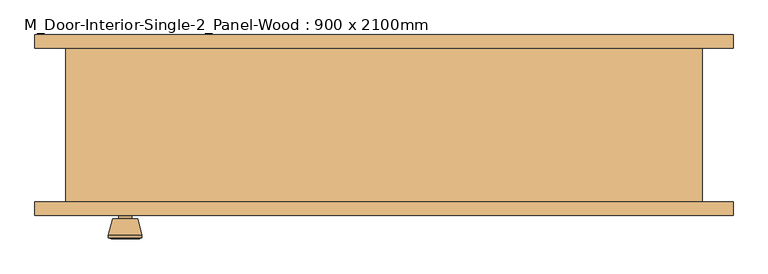
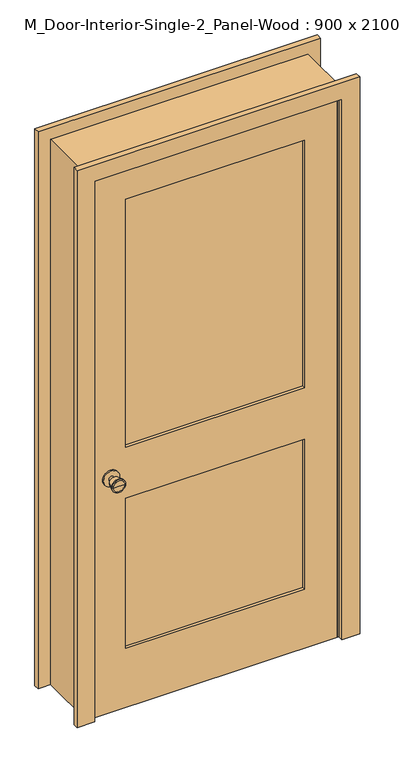
"""IFC4 building model written with IfcOpenShell, lengths in millimetres: door geometry, M_Door-Interior-Single-2_Panel-Wood : 900 x 2100mm."""

from ifc_helpers import new_model, si_unit, point, frame, frame_2d, origin, place, context, project, spatial, polyline, circle_curve, trimmed, segment, composite_curve, outline, extrude, faceted_brep, source, transform, mapped, element, save
from ifc_brep_helpers import plane_surface, cylinder_surface, revolved_surface, advanced_brep


def m_door_interior_single_2_panel_wood_900_x_2100mm_a85a1edd(model_context):
    return source(origin(), model_context, "Body", "SolidModel", [
        advanced_brep(
        [(-386.5, -70.825, 914.4), (-396.5, -70.825, 914.4), (-376.5, -70.825, 914.4), (-366.0241324, -21.825, 914.4), (-406.9758676, -21.825, 914.4), (-386.5, -21.825, 914.4), (-361.5, -23.6528681, 914.4), (-411.5, -23.6528681, 914.4), (-361.5, -27.1165463, 914.4), (-411.5, -27.1165463, 914.4), (-367.863764, -51.825, 914.4), (-405.136236, -51.825, 914.4), (-376.5, -51.825, 914.4), (-396.5, -51.825, 914.4)],
        [
            (0, 1),
            (1, 2, circle_curve(frame((-386.5, -70.825, 914.4), z_axis=(0.0, -1.0, 0.0), x_axis=(-1.0, 0.0, 0.0)), 10.0)),
            (2, 0),
            (2, 1, circle_curve(frame((-386.5, -70.825, 914.4), z_axis=(0.0, -1.0, 0.0), x_axis=(-1.0, 0.0, 0.0)), 10.0)),
            (3, 4, circle_curve(frame((-386.5, -21.825, 914.4), z_axis=(0.0, 1.0, 0.0), x_axis=(-1.0, 0.0, 0.0)), 20.4758676)),
            (4, 5),
            (5, 3),
            (4, 3, circle_curve(frame((-386.5, -21.825, 914.4), z_axis=(0.0, 1.0, 0.0), x_axis=(-1.0, 0.0, 0.0)), 20.4758676)),
            (6, 7, circle_curve(frame((-386.5, -23.6528681, 914.4), z_axis=(0.0, 1.0, 0.0), x_axis=(-1.0, 0.0, 0.0)), 25.0)),
            (7, 4),
            (3, 6),
            (7, 6, circle_curve(frame((-386.5, -23.6528681, 914.4), z_axis=(0.0, 1.0, 0.0), x_axis=(-1.0, 0.0, 0.0)), 25.0)),
            (8, 9, circle_curve(frame((-386.5, -27.1165463, 914.4), z_axis=(0.0, 1.0, 0.0), x_axis=(-1.0, 0.0, 0.0)), 25.0)),
            (9, 7),
            (6, 8),
            (9, 8, circle_curve(frame((-386.5, -27.1165463, 914.4), z_axis=(0.0, 1.0, 0.0), x_axis=(-1.0, 0.0, 0.0)), 25.0)),
            (10, 11, circle_curve(frame((-386.5, -51.825, 914.4), z_axis=(0.0, 1.0, 0.0), x_axis=(-1.0, 0.0, 0.0)), 18.636236)),
            (11, 9),
            (8, 10),
            (11, 10, circle_curve(frame((-386.5, -51.825, 914.4), z_axis=(0.0, 1.0, 0.0), x_axis=(-1.0, 0.0, 0.0)), 18.636236)),
            (12, 13, circle_curve(frame((-386.5, -51.825, 914.4), z_axis=(0.0, 1.0, 0.0), x_axis=(-1.0, 0.0, 0.0)), 10.0)),
            (13, 11),
            (10, 12),
            (13, 12, circle_curve(frame((-386.5, -51.825, 914.4), z_axis=(0.0, 1.0, 0.0), x_axis=(-1.0, 0.0, 0.0)), 10.0)),
            (1, 13),
            (12, 2),
        ],
        [
            plane_surface(frame((-386.5, -70.825, 914.4), z_axis=(0.0, -1.0, 0.0), x_axis=(-1.0, 0.0, 0.0))),
            plane_surface(frame((-386.5, -21.825, 914.4), z_axis=(0.0, 1.0, 0.0), x_axis=(-1.0, 0.0, 0.0))),
            revolved_surface(polyline([(-406.9758676, -21.825, 914.4), (-411.5, -23.6528681, 914.4)]), (-386.5, -70.825, 914.4), (0.0, -1.0, 0.0)),
            cylinder_surface(frame((-386.5, -70.825, 914.4), z_axis=(0.0, -1.0, 0.0), x_axis=(-1.0, 0.0, 0.0)), 25.0),
            revolved_surface(polyline([(-411.5, -27.1165463, 914.4), (-405.136236, -51.825, 914.4)]), (-386.5, -70.825, 914.4), (0.0, -1.0, 0.0)),
            plane_surface(frame((-386.5, -51.825, 914.4), z_axis=(0.0, -1.0, 0.0), x_axis=(-1.0, 0.0, 0.0))),
            cylinder_surface(frame((-386.5, -70.825, 914.4), z_axis=(0.0, -1.0, 0.0), x_axis=(-1.0, 0.0, 0.0)), 10.0),
        ],
        [
            (0, [[1, 2, 3]]),
            (0, [[-3, 4, -1]]),
            (1, [[5, 6, 7]]),
            (1, [[8, -7, -6]]),
            (2, [[9, 10, -5, 11]]),
            (2, [[12, -11, -8, -10]]),
            (3, [[13, 14, -9, 15]]),
            (3, [[16, -15, -12, -14]]),
            (4, [[17, 18, -13, 19]]),
            (4, [[20, -19, -16, -18]]),
            (5, [[21, 22, -17, 23]]),
            (5, [[24, -23, -20, -22]]),
            (6, [[-2, 25, -21, 26]]),
            (6, [[-4, -26, -24, -25]]),
        ],
    ),
        extrude(outline(composite_curve([segment(trimmed(circle_curve(frame_2d((914.4, -386.5)), 30.0), [point((914.4, -416.5))], [point((914.4, -356.5))], False, "CARTESIAN"), True, "CONTINUOUS"), segment(trimmed(circle_curve(frame_2d((914.4, -386.5)), 30.0), [point((914.4, -356.5))], [point((914.4, -416.5))], False, "CARTESIAN"), True, "CONTINUOUS")], self_intersect=False)), frame((0.0, -76.825, 0.0), z_axis=(0.0, 1.0, 0.0), x_axis=(0.0, 0.0, 1.0)), (0.0, 0.0, 1.0), 6.0),
        advanced_brep(
        [(-386.5, -117.825, 914.4), (-376.5, -117.825, 914.4), (-396.5, -117.825, 914.4), (-366.0241324, -166.825, 914.4), (-386.5, -166.825, 914.4), (-406.9758676, -166.825, 914.4), (-361.5, -164.9971319, 914.4), (-411.5, -164.9971319, 914.4), (-361.5, -161.5334537, 914.4), (-411.5, -161.5334537, 914.4), (-367.863764, -136.825, 914.4), (-405.136236, -136.825, 914.4), (-376.5, -136.825, 914.4), (-396.5, -136.825, 914.4)],
        [
            (0, 1),
            (1, 2, circle_curve(frame((-386.5, -117.825, 914.4), z_axis=(0.0, 1.0, 0.0), x_axis=(-1.0, 0.0, 0.0)), 10.0)),
            (2, 0),
            (2, 1, circle_curve(frame((-386.5, -117.825, 914.4), z_axis=(0.0, 1.0, 0.0), x_axis=(-1.0, 0.0, 0.0)), 10.0)),
            (3, 4),
            (4, 5),
            (5, 3, circle_curve(frame((-386.5, -166.825, 914.4), z_axis=(0.0, -1.0, 0.0), x_axis=(-1.0, 0.0, 0.0)), 20.4758676)),
            (3, 5, circle_curve(frame((-386.5, -166.825, 914.4), z_axis=(0.0, -1.0, 0.0), x_axis=(-1.0, 0.0, 0.0)), 20.4758676)),
            (6, 3),
            (5, 7),
            (7, 6, circle_curve(frame((-386.5, -164.9971319, 914.4), z_axis=(0.0, -1.0, 0.0), x_axis=(-1.0, 0.0, 0.0)), 25.0)),
            (6, 7, circle_curve(frame((-386.5, -164.9971319, 914.4), z_axis=(0.0, -1.0, 0.0), x_axis=(-1.0, 0.0, 0.0)), 25.0)),
            (8, 6),
            (7, 9),
            (9, 8, circle_curve(frame((-386.5, -161.5334537, 914.4), z_axis=(0.0, -1.0, 0.0), x_axis=(-1.0, 0.0, 0.0)), 25.0)),
            (8, 9, circle_curve(frame((-386.5, -161.5334537, 914.4), z_axis=(0.0, -1.0, 0.0), x_axis=(-1.0, 0.0, 0.0)), 25.0)),
            (10, 8),
            (9, 11),
            (11, 10, circle_curve(frame((-386.5, -136.825, 914.4), z_axis=(0.0, -1.0, 0.0), x_axis=(-1.0, 0.0, 0.0)), 18.636236)),
            (10, 11, circle_curve(frame((-386.5, -136.825, 914.4), z_axis=(0.0, -1.0, 0.0), x_axis=(-1.0, 0.0, 0.0)), 18.636236)),
            (12, 10),
            (11, 13),
            (13, 12, circle_curve(frame((-386.5, -136.825, 914.4), z_axis=(0.0, -1.0, 0.0), x_axis=(-1.0, 0.0, 0.0)), 10.0)),
            (12, 13, circle_curve(frame((-386.5, -136.825, 914.4), z_axis=(0.0, -1.0, 0.0), x_axis=(-1.0, 0.0, 0.0)), 10.0)),
            (1, 12),
            (13, 2),
        ],
        [
            plane_surface(frame((-386.5, -117.825, 914.4), z_axis=(0.0, 1.0, 0.0), x_axis=(-1.0, 0.0, 0.0))),
            plane_surface(frame((-386.5, -166.825, 914.4), z_axis=(0.0, -1.0, 0.0), x_axis=(-1.0, 0.0, 0.0))),
            revolved_surface(polyline([(-406.9758676, -166.825, 914.4), (-411.5, -164.9971319, 914.4)]), (-386.5, -117.825, 914.4), (0.0, 1.0, 0.0)),
            cylinder_surface(frame((-386.5, -117.825, 914.4), z_axis=(0.0, 1.0, 0.0), x_axis=(-1.0, 0.0, 0.0)), 25.0),
            revolved_surface(polyline([(-411.5, -161.5334537, 914.4), (-405.136236, -136.825, 914.4)]), (-386.5, -117.825, 914.4), (0.0, 1.0, 0.0)),
            plane_surface(frame((-386.5, -136.825, 914.4), z_axis=(0.0, 1.0, 0.0), x_axis=(-1.0, 0.0, 0.0))),
            cylinder_surface(frame((-386.5, -117.825, 914.4), z_axis=(0.0, 1.0, 0.0), x_axis=(-1.0, 0.0, 0.0)), 10.0),
        ],
        [
            (0, [[1, 2, 3]]),
            (0, [[-3, 4, -1]]),
            (1, [[5, 6, 7]]),
            (1, [[-6, -5, 8]]),
            (2, [[9, -7, 10, 11]]),
            (2, [[-10, -8, -9, 12]]),
            (3, [[13, -11, 14, 15]]),
            (3, [[-14, -12, -13, 16]]),
            (4, [[17, -15, 18, 19]]),
            (4, [[-18, -16, -17, 20]]),
            (5, [[21, -19, 22, 23]]),
            (5, [[-22, -20, -21, 24]]),
            (6, [[25, -23, 26, -2]]),
            (6, [[-26, -24, -25, -4]]),
        ],
    ),
        extrude(outline(composite_curve([segment(trimmed(circle_curve(frame_2d((914.4, -386.5)), 30.0), [point((914.4, -416.5))], [point((914.4, -356.5))], False, "CARTESIAN"), True, "CONTINUOUS"), segment(trimmed(circle_curve(frame_2d((914.4, -386.5)), 30.0), [point((914.4, -356.5))], [point((914.4, -416.5))], False, "CARTESIAN"), True, "CONTINUOUS")], self_intersect=False)), frame((0.0, -117.825, 0.0), z_axis=(0.0, 1.0, 0.0), x_axis=(0.0, 0.0, 1.0)), (0.0, 0.0, 1.0), 6.0),
        extrude(outline(polyline([(330.0, -88.4916667), (330.0, -100.1583333), (-330.0, -100.1583333), (-330.0, -88.4916667), (330.0, -88.4916667)])), frame((0.0, 0.0, 1014.4), z_axis=(0.0, 0.0, 1.0), x_axis=(1.0, 0.0, 0.0)), (0.0, 0.0, 1.0), 965.6),
        extrude(outline(polyline([(330.0, -88.4916667), (330.0, -100.1583333), (-330.0, -100.1583333), (-330.0, -88.4916667), (330.0, -88.4916667)])), frame((0.0, 0.0, 230.0), z_axis=(0.0, 0.0, 1.0), x_axis=(1.0, 0.0, 0.0)), (0.0, 0.0, 1.0), 584.4),
        extrude(outline(polyline([(2100.0, -450.0), (0.0, -450.0), (0.0, 450.0), (2100.0, 450.0), (2100.0, -450.0)]), holes=[polyline([(1980.0, -330.0), (1980.0, 330.0), (1014.4, 330.0), (1014.4, -330.0), (1980.0, -330.0)]), polyline([(814.4, -330.0), (814.4, 330.0), (230.0, 330.0), (230.0, -330.0), (814.4, -330.0)])]), frame((0.0, -111.825, 0.0), z_axis=(0.0, 1.0, 0.0), x_axis=(0.0, 0.0, 1.0)), (0.0, 0.0, 1.0), 35.0),
        faceted_brep([(475.0, -111.825, 0.0), (450.0, -111.825, 0.0), (450.0, -76.825, 0.0), (437.3, -76.825, 0.0), (437.3, -41.9, 0.0), (450.0, -41.9, 0.0), (450.0, 118.175, 0.0), (475.0, 118.175, 0.0), (475.0, 118.175, 2125.0), (475.0, -111.825, 2125.0), (450.0, 118.175, 2100.0), (-450.0, 118.175, 2100.0), (-450.0, 118.175, 0.0), (-475.0, 118.175, 0.0), (-475.0, 118.175, 2125.0), (450.0, -41.9, 2100.0), (437.3, -41.9, 2087.3), (-437.3, -41.9, 2087.3), (-437.3, -41.9, 0.0), (-450.0, -41.9, 0.0), (-450.0, -41.9, 2100.0), (437.3, -76.825, 2087.3), (450.0, -76.825, 2100.0), (-450.0, -76.825, 2100.0), (-450.0, -76.825, 0.0), (-437.3, -76.825, 0.0), (-437.3, -76.825, 2087.3), (450.0, -111.825, 2100.0), (-475.0, -111.825, 2125.0), (-475.0, -111.825, 0.0), (-450.0, -111.825, 0.0), (-450.0, -111.825, 2100.0)], [[[0, 1, 2, 3, 4, 5, 6, 7]], [[7, 8, 9, 0]], [[6, 10, 11, 12, 13, 14, 8, 7]], [[5, 15, 10, 6]], [[4, 16, 17, 18, 19, 20, 15, 5]], [[3, 21, 16, 4]], [[2, 22, 23, 24, 25, 26, 21, 3]], [[1, 27, 22, 2]], [[0, 9, 28, 29, 30, 31, 27, 1]], [[8, 14, 28, 9]], [[15, 20, 11, 10]], [[21, 26, 17, 16]], [[27, 31, 23, 22]], [[29, 13, 12, 19, 18, 25, 24, 30]], [[14, 13, 29, 28]], [[20, 19, 12, 11]], [[26, 25, 18, 17]], [[31, 30, 24, 23]]]),
        extrude(outline(polyline([(0.0, 521.35), (2171.35, 521.35), (2171.35, -521.35), (0.0, -521.35), (0.0, -456.35), (2106.35, -456.35), (2106.35, 456.35), (0.0, 456.35), (0.0, 521.35)])), frame((0.0, 118.175, 0.0), z_axis=(0.0, 1.0, 0.0), x_axis=(0.0, 0.0, 1.0)), (0.0, 0.0, 1.0), 20.0),
        extrude(outline(polyline([(0.0, 521.35), (2171.35, 521.35), (2171.35, -521.35), (0.0, -521.35), (0.0, -456.35), (2106.35, -456.35), (2106.35, 456.35), (0.0, 456.35), (0.0, 521.35)])), frame((0.0, -131.825, 0.0), z_axis=(0.0, 1.0, 0.0), x_axis=(0.0, 0.0, 1.0)), (0.0, 0.0, 1.0), 20.0),
    ])


if __name__ == "__main__":
    model = new_model("IFC4")
    model_context = context("Model", 3, world=origin())
    ifc_project = project(units=[si_unit("LENGTHUNIT", "METRE", prefix="MILLI")], contexts=[model_context])
    site = spatial("IfcSite", under=ifc_project)
    building = spatial("IfcBuilding", under=site)
    placement = place(None, origin())
    m_door_interior_single_2_panel_wood_900_x_2100mm_shape = m_door_interior_single_2_panel_wood_900_x_2100mm_a85a1edd(model_context)
    element("IfcDoor", 1, ObjectType="M_Door-Interior-Single-2_Panel-Wood : 900 x 2100mm", at=placement, inside=building, context=model_context, shape_type="MappedRepresentation", body=[
        mapped(m_door_interior_single_2_panel_wood_900_x_2100mm_shape, transform((0.0, 0.0, 0.0), x_axis=(1.0, 0.0, 0.0), y_axis=(0.0, 1.0, 0.0), z_axis=(0.0, 0.0, 1.0))),
    ])
    save(model, "model.ifc")

# Revit data of these elements
# Type "M_Door-Interior-Single-2_Panel-Wood : 900 x 2100mm"
#   Type Mark = "42"
#   Assembly Code = "C1020300"
#   Analytic Construction = "Wooden"
#   Top Rail = 12 cm
#   Thickness = 3.5 cm
#   Thermal Resistance (R) = 0.455703 (m²·K)/W
#   Swing Angle [instance default] = 90.00°
#   Stiles = 12 cm
#   Rough Width = 95 cm
#   Rough Height = 212.5 cm
#   Lock Rail = 20 cm
#   Height = 210 cm
#   Width = 90 cm
#   Heat Transfer Coefficient (U) = 2.19465 W/(m²·K)
#   Bottom Rail = 23 cm
#   Trim Material = Cherry
#   Panel Material = Cherry
#   Frame Material = Cherry
#   Door Handle Material = Aluminum
#   Visual Light Transmittance = 0
#   Solar Heat Gain Coefficient = 0
#   Wall Closure = (empty or 0)
#   Function = (empty or 0)
# Element 1 (IfcDoor, "M_Door-Interior-Single-2_Panel-Wood : 900 x 2100mm")
#   Materials on its faces: "Cherry", "Aluminum"
# Materials
#   "Cherry": class "Wood", colour RGB 226 177 128, transparency 0, Description = "Prunus Serotina", Cost = 0
#   "Aluminum": class "Metal", colour RGB 247 247 247, transparency 0, Description = "Aluminum 6061", Cost = 0
